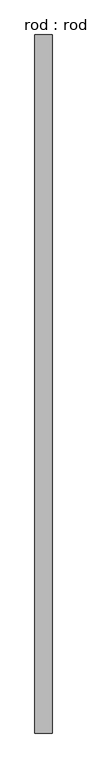
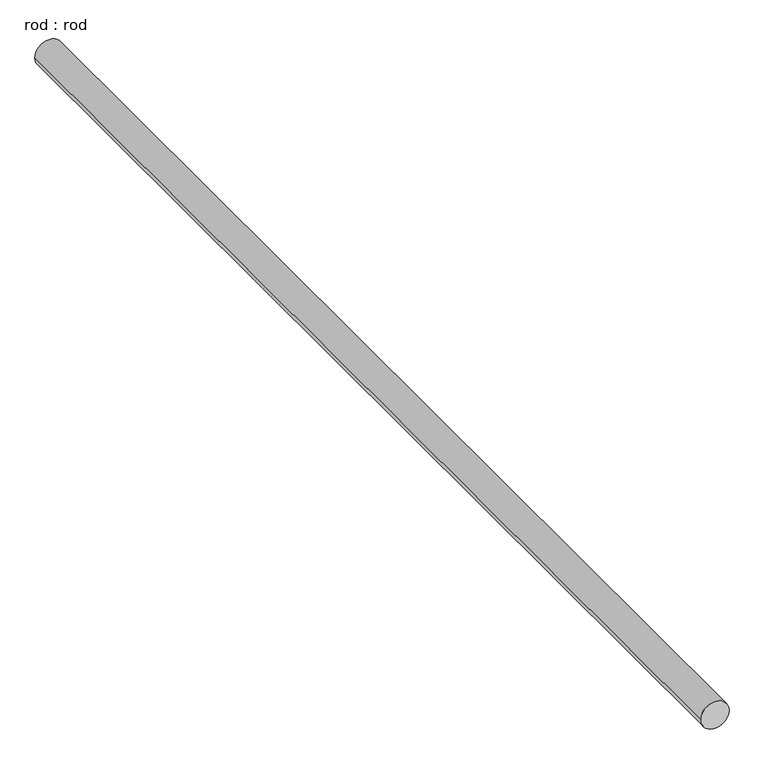
"""IFC4 building model written with IfcOpenShell, lengths in millimetres: proxy geometry, rod : rod."""

from ifc_helpers import new_model, si_unit, point, frame, frame_2d, origin, place, context, project, spatial, circle_curve, trimmed, segment, composite_curve, outline, extrude, source, transform, mapped, element, save


def rod_rod_62beb118(model_context):
    return source(origin(), model_context, "Body", "SweptSolid", [
        extrude(outline(composite_curve([segment(trimmed(circle_curve(frame_2d((0.0108462, 0.0)), 200.0), [point((0.0108462, 200.0))], [point((0.0108462, -200.0))], False, "CARTESIAN"), True, "CONTINUOUS"), segment(trimmed(circle_curve(frame_2d((0.0108462, 0.0)), 200.0), [point((0.0108462, -200.0))], [point((0.0108462, 200.0))], False, "CARTESIAN"), True, "CONTINUOUS")], self_intersect=False)), frame((0.0, -4039.1706397, 0.0), z_axis=(0.0, 1.0, 0.0), x_axis=(0.0, 0.0, 1.0)), (0.0, 0.0, 1.0), 16263.79851),
    ])


if __name__ == "__main__":
    model = new_model("IFC4")
    model_context = context("Model", 3, world=origin())
    ifc_project = project(units=[si_unit("LENGTHUNIT", "METRE", prefix="MILLI")], contexts=[model_context])
    site = spatial("IfcSite", under=ifc_project)
    building = spatial("IfcBuilding", under=site)
    placement = place(None, origin())
    rod_rod_shape = rod_rod_62beb118(model_context)
    element("IfcBuildingElementProxy", 1, Name="rod : rod", ObjectType="rod : rod", at=placement, inside=building, context=model_context, shape_type="MappedRepresentation", body=[
        mapped(rod_rod_shape, transform((0.0, 0.0, 0.0), x_axis=(1.0, 0.0, 0.0), y_axis=(0.0, 1.0, 0.0), z_axis=(0.0, 0.0, 1.0))),
    ])
    save(model, "model.ifc")

# Revit data of these elements
# Type "rod : rod"
#   Default Elevation = 0
